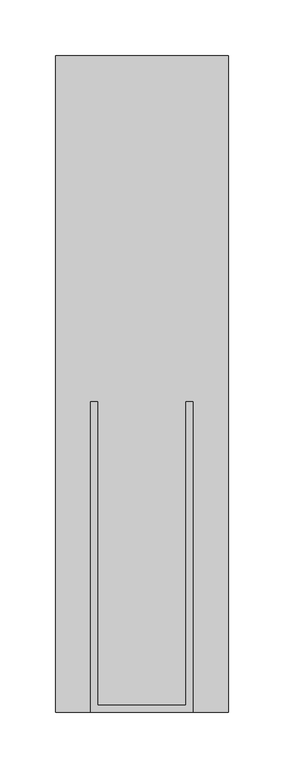
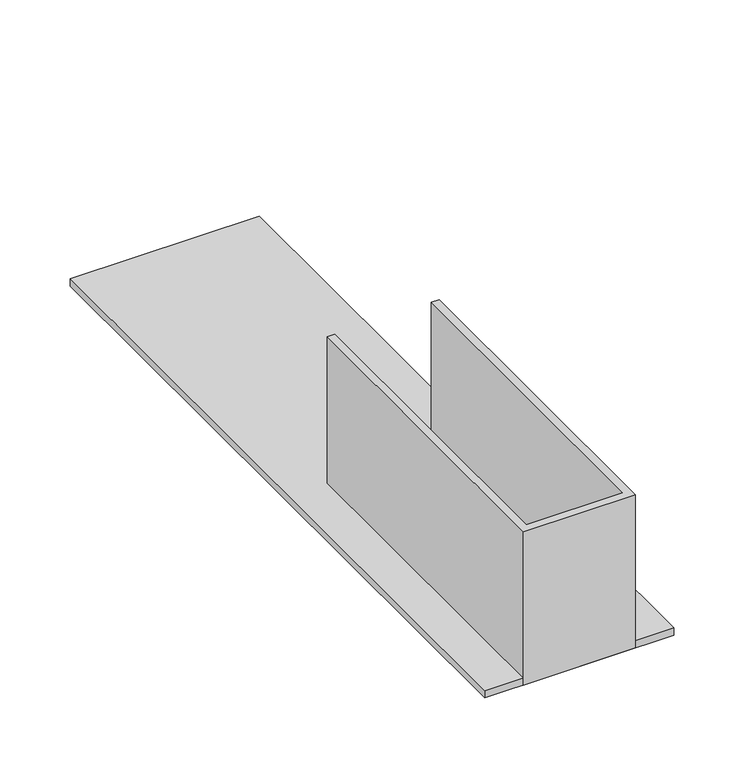
"""IFC4 building model written with IfcOpenShell, lengths in millimetres: fastener geometry, SIMPSON -THGBV - Truss Girder Hanger : SIMPSON -THGBV3.62/11 - HDG."""

from ifc_helpers import new_model, si_unit, origin, origin_with_axes, place, context, project, spatial, polyline, outline, extrude, source, transform, mapped, element, save


def fastener_a0b837a1(model_context):
    return source(origin(), model_context, "Body", "SweptSolid", [
        extrude(outline(polyline([(-46.0375, 0.0), (-46.0375, 279.4), (-39.6875, 279.4), (-39.6875, 6.35), (39.6875, 6.35), (39.6875, 279.4), (46.0375, 279.4), (46.0375, 0.0), (-46.0375, 0.0)])), origin_with_axes(), (0.0, 0.0, 1.0), 133.35),
        extrude(outline(polyline([(77.7875, 590.55), (77.7875, 0.0), (-77.7875, 0.0), (-77.7875, 590.55), (77.7875, 590.55)])), origin_with_axes(), (0.0, 0.0, 1.0), 6.35),
    ])


if __name__ == "__main__":
    model = new_model("IFC4")
    model_context = context("Model", 3, world=origin())
    ifc_project = project(units=[si_unit("LENGTHUNIT", "METRE", prefix="MILLI")], contexts=[model_context])
    site = spatial("IfcSite", under=ifc_project)
    building = spatial("IfcBuilding", under=site)
    placement = place(None, origin())
    fastener_shape = fastener_a0b837a1(model_context)
    element("IfcFastener", 1, ObjectType="SIMPSON -THGBV - Truss Girder Hanger : SIMPSON -THGBV3.62/11 - HDG", at=placement, inside=building, context=model_context, shape_type="MappedRepresentation", body=[
        mapped(fastener_shape, transform((0.0, 0.0, 0.0), x_axis=(1.0, 0.0, 0.0), y_axis=(0.0, 1.0, 0.0), z_axis=(0.0, 0.0, 1.0))),
    ])
    save(model, "model.ifc")

# Revit data of these elements
# Type "SIMPSON -THGBV - Truss Girder Hanger : SIMPSON -THGBV3.62/11 - HDG"
#   URL = "http://embed.widencdn.net/pdf/plus/ssttoolbox/iecrxc4cbv/C-C-2017-p254-255.pdf"
#   W = 0' - 3 5/8"
#   H = 0' - 11"
#   Default Elevation = 4' - 0"
